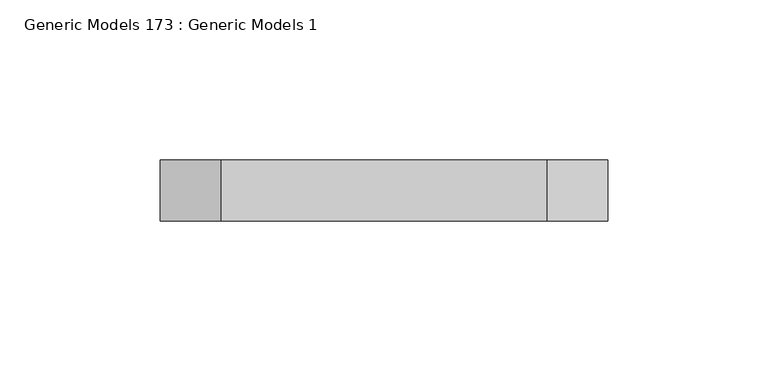
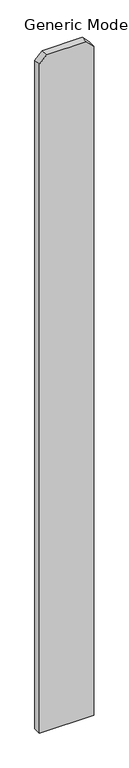
"""IFC4 building model written with IfcOpenShell, lengths in millimetres: proxy geometry, Generic Models 173 : Generic Models 1."""

import ifcopenshell
import ifcopenshell.guid

model = None  # the IFC model being written
_history = None  # IfcOwnerHistory: only IFC2X3 demands one
_inside = {}  # id of a spatial element -> (the spatial element, [elements in it])
_under = {}  # id of a project, library or spatial element -> (it, [spatial elements below it])
_declared = {}  # id of a project -> (the project, [libraries it declares])
_typed = {}  # id of a type object -> (the type object, [elements of that type])
_made_of = {}  # id of a material, layer set ... -> (it, [elements and type objects made of it])


def new_model(schema):
    """Start an empty IFC model of exactly this schema.

    Asked for "IFC4X3", IfcOpenShell would pick the latest addendum, in which some entities
    have other attributes; the version numbers below select the first issue.
    IFC2X3 requires an IfcOwnerHistory on every rooted entity: one is made here for all.
    """
    global model, _history
    if schema == "IFC4X3":
        model = ifcopenshell.file(schema_version=(4, 3, 0, 0))
    else:
        model = ifcopenshell.file(schema=schema)
    _inside.clear()
    _under.clear()
    _declared.clear()
    _typed.clear()
    _made_of.clear()
    _history = None
    if model.schema == "IFC2X3":
        org = make("IfcOrganization", Name="unknown")
        user = make(
            "IfcPersonAndOrganization",
            ThePerson=make("IfcPerson", FamilyName="unknown"),
            TheOrganization=org,
        )
        app = make(
            "IfcApplication",
            ApplicationDeveloper=org,
            Version="unknown",
            ApplicationFullName="unknown",
            ApplicationIdentifier="unknown",
        )
        _history = make(
            "IfcOwnerHistory",
            OwningUser=user,
            OwningApplication=app,
            ChangeAction="ADDED",
            CreationDate=0,
        )
    return model


def make(cls, **values):
    """One entity of the class cls with the attributes given. An attribute that is None is left unset."""
    return model.create_entity(
        cls, **{name: value for name, value in values.items() if value is not None}
    )


def rooted(cls, **values):
    """An entity with a GlobalId (a new one), such as an element, a storey or a relation."""
    return make(cls, GlobalId=ifcopenshell.guid.new(), OwnerHistory=_history, **values)


def si_unit(unit_type, name, prefix=None):
    """IfcSIUnit, for example si_unit("LENGTHUNIT", "METRE", prefix="MILLI")."""
    return make("IfcSIUnit", UnitType=unit_type, Prefix=prefix, Name=name)


def assignment(units):
    """IfcUnitAssignment: the units of a project."""
    return None if units is None else make("IfcUnitAssignment", Units=units)


def point(xyz):
    """IfcCartesianPoint."""
    return None if xyz is None else make("IfcCartesianPoint", Coordinates=xyz)


def direction(xyz):
    """IfcDirection."""
    return None if xyz is None else make("IfcDirection", DirectionRatios=xyz)


def frame(location, z_axis=None, x_axis=None):
    """IfcAxis2Placement3D, a coordinate frame: its origin and axes. An axis left out is left unset."""
    return make(
        "IfcAxis2Placement3D",
        Location=point(location),
        Axis=direction(z_axis),
        RefDirection=direction(x_axis),
    )


def origin():
    """The frame at (0, 0, 0) with its axes left unset."""
    return frame((0.0, 0.0, 0.0))


def place(relative_to, where):
    """IfcLocalPlacement: puts the frame where relative to a parent placement (None: the world)."""
    return make(
        "IfcLocalPlacement", PlacementRelTo=relative_to, RelativePlacement=where
    )


def context(
    kind, dimensions, precision=None, world=None, true_north=None, identifier=None
):
    """IfcGeometricRepresentationContext, for example the 3D "Model" context."""
    return make(
        "IfcGeometricRepresentationContext",
        ContextIdentifier=identifier,
        ContextType=kind,
        CoordinateSpaceDimension=dimensions,
        Precision=precision,
        WorldCoordinateSystem=world,
        TrueNorth=true_north,
    )


def project(units=None, contexts=None):
    """IfcProject with its units and contexts."""
    return rooted(
        "IfcProject",
        Name="project",
        RepresentationContexts=contexts,
        UnitsInContext=assignment(units),
    )


def spatial(cls, under=None, at=None, **own):
    """A site, building, storey or space (cls), placed at a placement, below another one or the project."""
    s = rooted(cls, ObjectPlacement=at, **own)
    if under is not None:
        _under.setdefault(under.id(), (under, []))[1].append(s)
    return s


def polyline(points):
    """IfcPolyline through the points."""
    return make("IfcPolyline", Points=[point(p) for p in points])


def outline(outer, holes=None, kind="AREA"):
    """IfcArbitraryClosedProfileDef: a profile drawn as a closed curve; with holes, ...WithVoids."""
    if holes is None:
        return make("IfcArbitraryClosedProfileDef", ProfileType=kind, OuterCurve=outer)
    return make(
        "IfcArbitraryProfileDefWithVoids",
        ProfileType=kind,
        OuterCurve=outer,
        InnerCurves=holes,
    )


def extrude(swept, where, along, depth):
    """IfcExtrudedAreaSolid: the profile swept, set in the frame where, extruded along a direction by depth."""
    return make(
        "IfcExtrudedAreaSolid",
        SweptArea=swept,
        Position=where,
        ExtrudedDirection=direction(along),
        Depth=depth,
    )


def shape(context_of_items, identifier, shape_type, items):
    """IfcShapeRepresentation: the items that make up one representation, for example the "Body"."""
    return make(
        "IfcShapeRepresentation",
        ContextOfItems=context_of_items,
        RepresentationIdentifier=identifier,
        RepresentationType=shape_type,
        Items=items,
    )


def source(mapping_origin, context_of_items, identifier, shape_type, items):
    """IfcRepresentationMap: a shape defined once, which mapped items show again and again."""
    return make(
        "IfcRepresentationMap",
        MappingOrigin=mapping_origin,
        MappedRepresentation=shape(context_of_items, identifier, shape_type, items),
    )


def transform(
    local_origin,
    x_axis=None,
    y_axis=None,
    z_axis=None,
    scale=None,
    scale2=None,
    scale3=None,
    uniform=True,
):
    """IfcCartesianTransformationOperator3D, or its non-uniform kind. x_axis, y_axis, z_axis: its Axis1, 2, 3."""
    if uniform:
        return make(
            "IfcCartesianTransformationOperator3D",
            Axis1=direction(x_axis),
            Axis2=direction(y_axis),
            LocalOrigin=point(local_origin),
            Scale=scale,
            Axis3=direction(z_axis),
        )
    return make(
        "IfcCartesianTransformationOperator3DnonUniform",
        Axis1=direction(x_axis),
        Axis2=direction(y_axis),
        LocalOrigin=point(local_origin),
        Scale=scale,
        Axis3=direction(z_axis),
        Scale2=scale2,
        Scale3=scale3,
    )


def mapped(mapping_source, mapping_target):
    """IfcMappedItem: shows the shape of a source again, moved by a transform."""
    return make(
        "IfcMappedItem", MappingSource=mapping_source, MappingTarget=mapping_target
    )


def made_of(thing, what):
    """Note that an element or type object is made of a material, layer set ...; save() writes the relation."""
    if what is not None:
        _made_of.setdefault(what.id(), (what, []))[1].append(thing)
    return thing


def element(
    cls,
    number,
    at=None,
    inside=None,
    cuts=None,
    type_object=None,
    material=None,
    context=None,
    identifier="Body",
    shape_type=None,
    held_by="IfcProductDefinitionShape",
    body=None,
    shapes=None,
    **own,
):
    """One element of the class cls, such as IfcWall. Its Tag is "e" and its number.

    at: its placement. inside: the storey or other place that contains it. cuts: it is an
    opening in that element (IfcRelVoidsElement). A single representation is given by context,
    identifier, shape_type and body (its items); several are given by shapes. held_by: the class
    of the entity that holds the representations. save() writes the other relations.
    """
    e = rooted(cls, Tag="e%d" % number, ObjectPlacement=at, **own)
    if body is not None:
        shapes = [shape(context, identifier, shape_type, body)]
    if shapes is not None:
        e.Representation = make(held_by, Representations=shapes)
    if inside is not None:
        _inside.setdefault(inside.id(), (inside, []))[1].append(e)
    if cuts is not None:
        rooted(
            "IfcRelVoidsElement", RelatingBuildingElement=cuts, RelatedOpeningElement=e
        )
    if type_object is not None:
        _typed.setdefault(type_object.id(), (type_object, []))[1].append(e)
    return made_of(e, material)


def aggregate(whole, parts):
    """IfcRelAggregates: a whole, such as a stair, and the parts it consists of."""
    return rooted("IfcRelAggregates", RelatingObject=whole, RelatedObjects=parts)


def save(model, path):
    """Write the relations noted so far, then the file.

    IfcRelAggregates (storeys below a building ...), IfcRelContainedInSpatialStructure (elements
    in a storey), IfcRelDefinesByType, IfcRelAssociatesMaterial and IfcRelDeclares: one each for
    every whole, place, type object, material and project.
    """
    for whole, parts in _under.values():
        aggregate(whole, parts)
    for where, things in _inside.values():
        rooted(
            "IfcRelContainedInSpatialStructure",
            RelatedElements=things,
            RelatingStructure=where,
        )
    for kind, things in _typed.values():
        rooted("IfcRelDefinesByType", RelatedObjects=things, RelatingType=kind)
    for what, things in _made_of.values():
        rooted("IfcRelAssociatesMaterial", RelatedObjects=things, RelatingMaterial=what)
    for by, libraries in _declared.values():
        rooted("IfcRelDeclares", RelatingContext=by, RelatedDefinitions=libraries)
    model.write(path)


def generic_models_173_generic_models_1_7547f4db(model_context):
    return source(origin(), model_context, "Body", "SweptSolid", [
        extrude(outline(polyline([(76.2, 56361.0125), (1885.95, 56361.0125), (1905.0, 56341.9625), (1905.0, 56240.3625), (1885.95, 56221.3125), (76.2, 56221.3125), (76.2, 56361.0125)])), frame((0.0, 547.6875, 0.0), z_axis=(0.0, 1.0, 0.0), x_axis=(0.0, 0.0, 1.0)), (0.0, 0.0, 1.0), 19.05),
    ])


if __name__ == "__main__":
    model = new_model("IFC4")
    model_context = context("Model", 3, world=origin())
    ifc_project = project(units=[si_unit("LENGTHUNIT", "METRE", prefix="MILLI")], contexts=[model_context])
    site = spatial("IfcSite", under=ifc_project)
    building = spatial("IfcBuilding", under=site)
    placement = place(None, origin())
    generic_models_173_generic_models_1_shape = generic_models_173_generic_models_1_7547f4db(model_context)
    element("IfcBuildingElementProxy", 1, Name="Generic Models 173 : Generic Models 1", ObjectType="Generic Models 173 : Generic Models 1", at=placement, inside=building, context=model_context, shape_type="MappedRepresentation", body=[
        mapped(generic_models_173_generic_models_1_shape, transform((0.0, 0.0, 0.0), x_axis=(1.0, 0.0, 0.0), y_axis=(0.0, 1.0, 0.0), z_axis=(0.0, 0.0, 1.0))),
    ])
    save(model, "model.ifc")

# Revit data of these elements
# Element 1 (IfcBuildingElementProxy, "Generic Models 173 : Generic Models 1")
#   Materials on its faces: "VERTICAL 1X6 CEDAR PLANKS W/ CLEAR WOOD SEALER"
# Materials
#   "VERTICAL 1X6 CEDAR PLANKS W/ CLEAR WOOD SEALER": class "Wood", colour RGB 234 198 147, transparency 0, Description = "Pinus Echinata", Cost = 0
